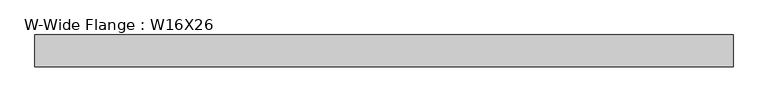
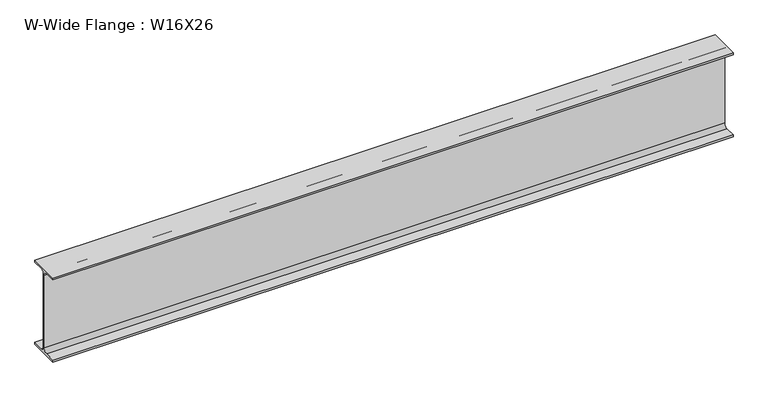
"""IFC4 building model written with IfcOpenShell, lengths in millimetres: beam geometry, W-Wide Flange : W16X26."""

from ifc_helpers import new_model, si_unit, point, frame, frame_2d, origin, place, context, project, spatial, polyline, circle_curve, trimmed, segment, composite_curve, outline, extrude, source, transform, mapped, element, save


def w_wide_flange_w16x26_2b48321a(model_context):
    return source(origin(), model_context, "Body", "SweptSolid", [
        extrude(outline(composite_curve([segment(polyline([(69.85, -190.627), (69.85, -199.39), (-69.85, -199.39), (-69.85, -190.627), (-21.3995, -190.627)]), True, "CONTINUOUS"), segment(trimmed(circle_curve(frame_2d((-21.3995, -172.4025)), 18.2245), [point((-21.3995, -190.627))], [point((-3.175, -172.4025))], True, "CARTESIAN"), True, "CONTINUOUS"), segment(polyline([(-3.175, -172.4025), (-3.175, 172.4025)]), True, "CONTINUOUS"), segment(trimmed(circle_curve(frame_2d((-21.3995, 172.4025)), 18.2245), [point((-3.175, 172.4025))], [point((-21.3995, 190.627))], True, "CARTESIAN"), True, "CONTINUOUS"), segment(polyline([(-21.3995, 190.627), (-69.85, 190.627), (-69.85, 199.39), (69.85, 199.39), (69.85, 190.627), (21.3995, 190.627)]), True, "CONTINUOUS"), segment(trimmed(circle_curve(frame_2d((21.3995, 172.4025)), 18.2245), [point((21.3995, 190.627))], [point((3.175, 172.4025))], True, "CARTESIAN"), True, "CONTINUOUS"), segment(polyline([(3.175, 172.4025), (3.175, -172.4025)]), True, "CONTINUOUS"), segment(trimmed(circle_curve(frame_2d((21.3995, -172.4025)), 18.2245), [point((3.175, -172.4025))], [point((21.3995, -190.627))], True, "CARTESIAN"), True, "CONTINUOUS"), segment(polyline([(21.3995, -190.627), (69.85, -190.627)]), True, "CONTINUOUS")], self_intersect=False)), frame((-1565.0792965, 0.0, 0.0), z_axis=(1.0, 0.0, 0.0), x_axis=(0.0, 1.0, 0.0)), (0.0, 0.0, 1.0), 3053.9771006),
    ])


if __name__ == "__main__":
    model = new_model("IFC4")
    model_context = context("Model", 3, world=origin())
    ifc_project = project(units=[si_unit("LENGTHUNIT", "METRE", prefix="MILLI")], contexts=[model_context])
    site = spatial("IfcSite", under=ifc_project)
    building = spatial("IfcBuilding", under=site)
    placement = place(None, origin())
    w_wide_flange_w16x26_shape = w_wide_flange_w16x26_2b48321a(model_context)
    element("IfcBeam", 1, ObjectType="W-Wide Flange : W16X26", at=placement, inside=building, context=model_context, shape_type="MappedRepresentation", body=[
        mapped(w_wide_flange_w16x26_shape, transform((0.0, 0.0, 0.0), x_axis=(1.0, 0.0, 0.0), y_axis=(0.0, 1.0, 0.0), z_axis=(0.0, 0.0, 1.0))),
    ])
    save(model, "model.ifc")

# Revit data of these elements
# Type "W-Wide Flange : W16X26"
#   Assembly Code = "B10"
#   W = 26
#   Length [instance default] = 5' - 0"
#   bf = 0' - 5 1/2"
#   d = 1' - 3.7"
#   k = 0' - 1 1/16"
#   k2 = 0' - 0.7175"
#   tf = 0' - 0.345"
#   tw = 0' - 0 1/4"
#   A = 0.0533333 SF
#   Structural Material [instance default] = Steel ASTM A992
# Element 1 (IfcBeam, "W-Wide Flange : W16X26")
#   Structural Material = Steel ASTM A36
#   Materials on its faces: "Steel ASTM A36"
# Materials
#   "Steel ASTM A992": class "Metal", colour RGB 199 199 199, transparency 0, Description = "Structural steel 50ksi", Cost = 0
#   "Steel ASTM A36": class "Metal", colour RGB 199 199 199, transparency 0, Description = "Structural steel, ASTM A36 Grade B, mill finish", Cost = 0
